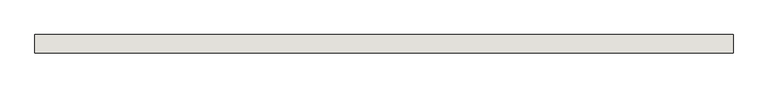
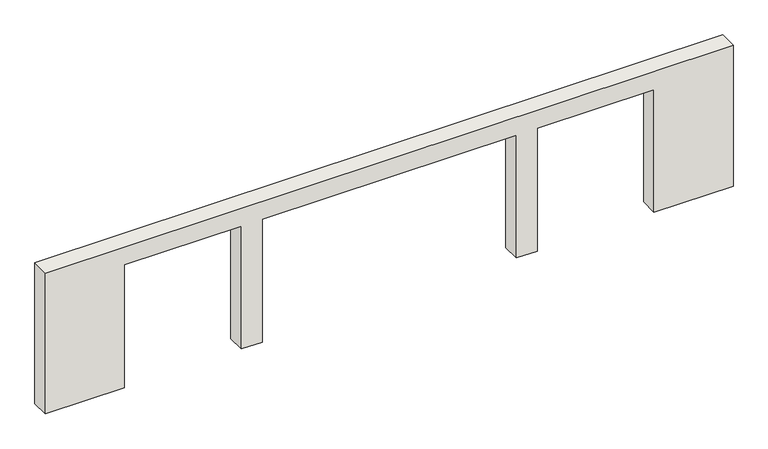
"""IFC4 building model written with IfcOpenShell, lengths in millimetres: wall geometry, 0_3d_modell."""

from ifc_helpers import new_model, si_unit, frame, origin, place, context, project, spatial, polyline, outline, extrude, source, transform, mapped, element, save


def wall_89b89b3e(model_context):
    return source(origin(), model_context, "Body", "SweptSolid", [
        extrude(outline(polyline([(2510.0, 11770.0), (0.0, 11770.0), (0.0, 13300.0), (2880.0, 13300.0), (2880.0, 0.0), (0.0, 0.0), (0.0, 1530.0), (2510.0, 1530.0), (2510.0, 3790.0), (0.0, 3790.0), (0.0, 4190.0), (2510.0, 4190.0), (2510.0, 9110.0), (0.0, 9110.0), (0.0, 9510.0), (2510.0, 9510.0), (2510.0, 11770.0)])), frame((0.0, 0.0, 0.0), z_axis=(0.0, 1.0, 0.0), x_axis=(0.0, 0.0, 1.0)), (0.0, 0.0, 1.0), 350.0),
    ])


if __name__ == "__main__":
    model = new_model("IFC4")
    model_context = context("Model", 3, world=origin())
    ifc_project = project(units=[si_unit("LENGTHUNIT", "METRE", prefix="MILLI")], contexts=[model_context])
    site = spatial("IfcSite", under=ifc_project)
    building = spatial("IfcBuilding", under=site)
    placement = place(None, origin())
    wall_shape = wall_89b89b3e(model_context)
    element("IfcWall", 1, ObjectType="0_3d_modell", at=placement, inside=building, context=model_context, shape_type="MappedRepresentation", body=[
        mapped(wall_shape, transform((0.0, 0.0, 0.0), x_axis=(1.0, 0.0, 0.0), y_axis=(0.0, 1.0, 0.0), z_axis=(0.0, 0.0, 1.0))),
    ])
    save(model, "model.ifc")

# Revit data of these elements
# Element 1 (IfcWall, "0_3d_modell")
#   Materials on its faces: "holzschalung"
# Materials
#   "holzschalung": class "Unassigned", colour RGB 128 128 128, transparency 0
